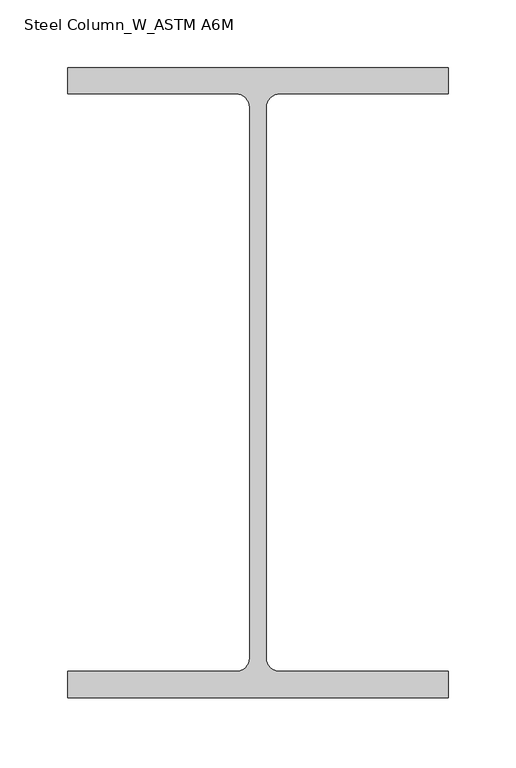
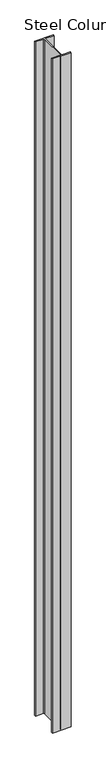
"""IFC4 building model written with IfcOpenShell, lengths in millimetres: column geometry, Steel Column_W_ASTM A6M : H_SC_AR_S01_W460x128_C1."""

from ifc_helpers import new_model, si_unit, point, frame, frame_2d, origin, place, context, project, spatial, polyline, circle_curve, trimmed, segment, composite_curve, outline, extrude, source, transform, mapped, element, save


def steel_column_w_astm_a6m_c7f0337f(model_context):
    return source(origin(), model_context, "Body", "SweptSolid", [
        extrude(outline(composite_curve([segment(polyline([(141.0, 233.5), (141.0, 213.9), (16.2, 213.9)]), True, "CONTINUOUS"), segment(trimmed(circle_curve(frame_2d((16.2, 203.8)), 10.1), [point((16.2, 213.9))], [point((6.1, 203.8))], True, "CARTESIAN"), True, "CONTINUOUS"), segment(polyline([(6.1, 203.8), (6.1, -203.8)]), True, "CONTINUOUS"), segment(trimmed(circle_curve(frame_2d((16.2, -203.8)), 10.1), [point((6.1, -203.8))], [point((16.2, -213.9))], True, "CARTESIAN"), True, "CONTINUOUS"), segment(polyline([(16.2, -213.9), (141.0, -213.9), (141.0, -233.5), (-141.0, -233.5), (-141.0, -213.9), (-16.2, -213.9)]), True, "CONTINUOUS"), segment(trimmed(circle_curve(frame_2d((-16.2, -203.8)), 10.1), [point((-16.2, -213.9))], [point((-6.1, -203.8))], True, "CARTESIAN"), True, "CONTINUOUS"), segment(polyline([(-6.1, -203.8), (-6.1, 203.8)]), True, "CONTINUOUS"), segment(trimmed(circle_curve(frame_2d((-16.2, 203.8)), 10.1), [point((-6.1, 203.8))], [point((-16.2, 213.9))], True, "CARTESIAN"), True, "CONTINUOUS"), segment(polyline([(-16.2, 213.9), (-141.0, 213.9), (-141.0, 233.5), (141.0, 233.5)]), True, "CONTINUOUS")], self_intersect=False)), frame((0.0, 0.0, -7269.1756499), z_axis=(0.0, 0.0, 1.0), x_axis=(1.0, 0.0, 0.0)), (0.0, 0.0, 1.0), 10789.0),
    ])


if __name__ == "__main__":
    model = new_model("IFC4")
    model_context = context("Model", 3, world=origin())
    ifc_project = project(units=[si_unit("LENGTHUNIT", "METRE", prefix="MILLI")], contexts=[model_context])
    site = spatial("IfcSite", under=ifc_project)
    building = spatial("IfcBuilding", under=site)
    placement = place(None, origin())
    steel_column_w_astm_a6m_shape = steel_column_w_astm_a6m_c7f0337f(model_context)
    element("IfcColumn", 1, ObjectType="Steel Column_W_ASTM A6M : H_SC_AR_S01_W460x128_C1", at=placement, inside=building, context=model_context, shape_type="MappedRepresentation", body=[
        mapped(steel_column_w_astm_a6m_shape, transform((0.0, 0.0, 0.0), x_axis=(1.0, 0.0, 0.0), y_axis=(0.0, 1.0, 0.0), z_axis=(0.0, 0.0, 1.0))),
    ])
    save(model, "model.ifc")

# Revit data of these elements
# Type "Steel Column_W_ASTM A6M : H_SC_AR_S01_W460x128_C1"
#   Section Name Key = "W18x86"
#   Width = 28.2 cm
#   Web Thickness = 1.22 cm
#   Web Fillet = 1.01 cm
#   Warping Constant = 3650000.0 cm⁶
#   Torsional Moment of Inertia = 171.00 cm⁴
#   Section Area = 163.0 cm²
#   Plastic Modulus weak axis = 793.0 cm³
#   Plastic Modulus strong axis = 3050.0 cm³
#   Perimeter = 2.02 m²/m
#   Nominal Weight = 128.00 kgf/m
#   Moment of Inertia weak axis = 7280.00 cm⁴
#   Moment of Inertia strong axis = 63700.00 cm⁴
#   Height = 46.7 cm
#   Flange Thickness = 1.96 cm
#   Elastic Modulus weak axis = 518.0 cm³
#   Elastic Modulus strong axis = 2720.0 cm³
#   Centroid Vertical = 23.35 cm
#   Centroid Horizontal = 14.1 cm
#   Structural Material [instance default] = Steel, 45-345
#   Bolt Spacing = 0
#   Assembly Code = ""
# Element 1 (IfcColumn, "Steel Column_W_ASTM A6M : H_SC_AR_S01_W460x128_C1")
#   Structural Material = Steel ASTM A992 GRADE 50
#   Materials on its faces: "Steel ASTM A992 GRADE 50"
# Materials
#   "Steel, 45-345": class "Metal", colour RGB 189 187 185, transparency 0, Description = "Steel 345 MPa", Cost = 0
#   "Steel ASTM A992 GRADE 50": class "Metal", colour RGB 120 120 120, transparency 0, Description = "Structural steel 50ksi", Cost = 0
